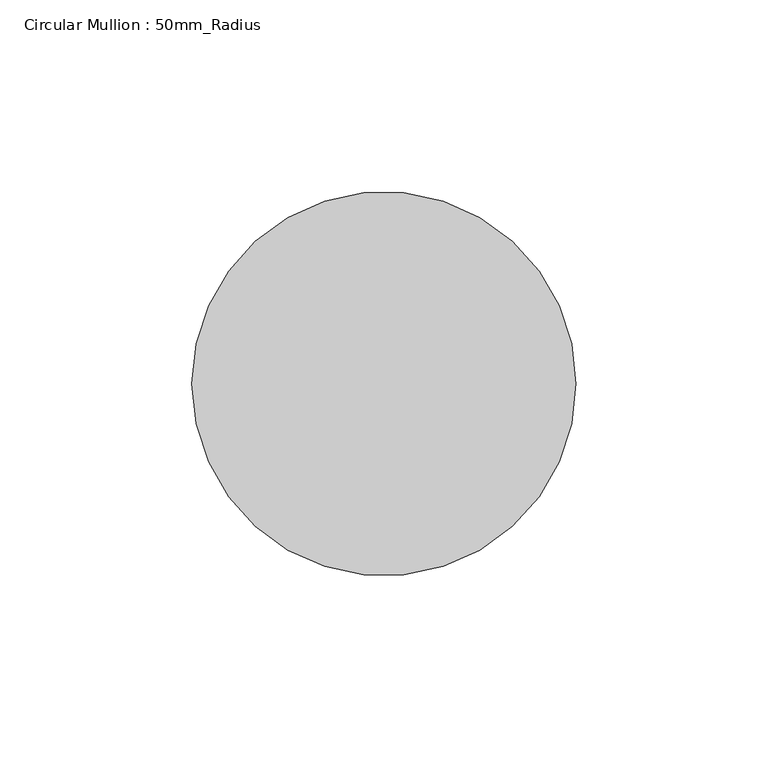
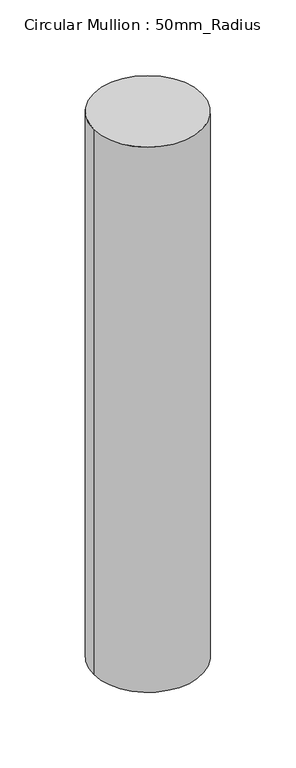
"""IFC4 building model written with IfcOpenShell, lengths in millimetres: member geometry, Circular Mullion : 50mm_Radius."""

from ifc_helpers import new_model, si_unit, point, frame, origin, origin_2d, place, context, project, spatial, circle_curve, trimmed, segment, composite_curve, outline, extrude, source, transform, mapped, element, save


def circular_mullion_50mm_radius_fbcd57ac(model_context):
    return source(origin(), model_context, "Body", "SweptSolid", [
        extrude(outline(composite_curve([segment(trimmed(circle_curve(origin_2d(), 50.0), [point((50.0, 0.0))], [point((-50.0, 0.0))], False, "CARTESIAN"), True, "CONTINUOUS"), segment(trimmed(circle_curve(origin_2d(), 50.0), [point((-50.0, 0.0))], [point((50.0, 0.0))], False, "CARTESIAN"), True, "CONTINUOUS")], self_intersect=False)), frame((0.0, 0.0, -532.5), z_axis=(0.0, 0.0, 1.0), x_axis=(1.0, 0.0, 0.0)), (0.0, 0.0, 1.0), 532.5),
    ])


if __name__ == "__main__":
    model = new_model("IFC4")
    model_context = context("Model", 3, world=origin())
    ifc_project = project(units=[si_unit("LENGTHUNIT", "METRE", prefix="MILLI")], contexts=[model_context])
    site = spatial("IfcSite", under=ifc_project)
    building = spatial("IfcBuilding", under=site)
    placement = place(None, origin())
    circular_mullion_50mm_radius_shape = circular_mullion_50mm_radius_fbcd57ac(model_context)
    element("IfcMember", 1, ObjectType="Circular Mullion : 50mm_Radius", at=placement, inside=building, context=model_context, shape_type="MappedRepresentation", body=[
        mapped(circular_mullion_50mm_radius_shape, transform((0.0, 0.0, 0.0), x_axis=(1.0, 0.0, 0.0), y_axis=(0.0, 1.0, 0.0), z_axis=(0.0, 0.0, 1.0))),
    ])
    save(model, "model.ifc")

# Revit data of these elements
# Type "Circular Mullion : 50mm_Radius"
#   Keynote = "H11"
#   built-in parameter 1007350 = 0.164042 (stored number, unit not read)
# Element 1 (IfcMember, "Circular Mullion : 50mm_Radius")
#   Materials on its faces: "Aluminium"
# Materials
#   "Aluminium": class "Metal", colour RGB 247 247 247, transparency 0, Description = "Aluminium 6061", Cost = 0
